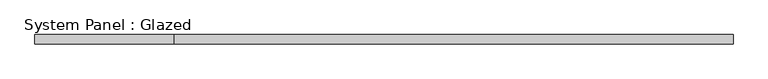
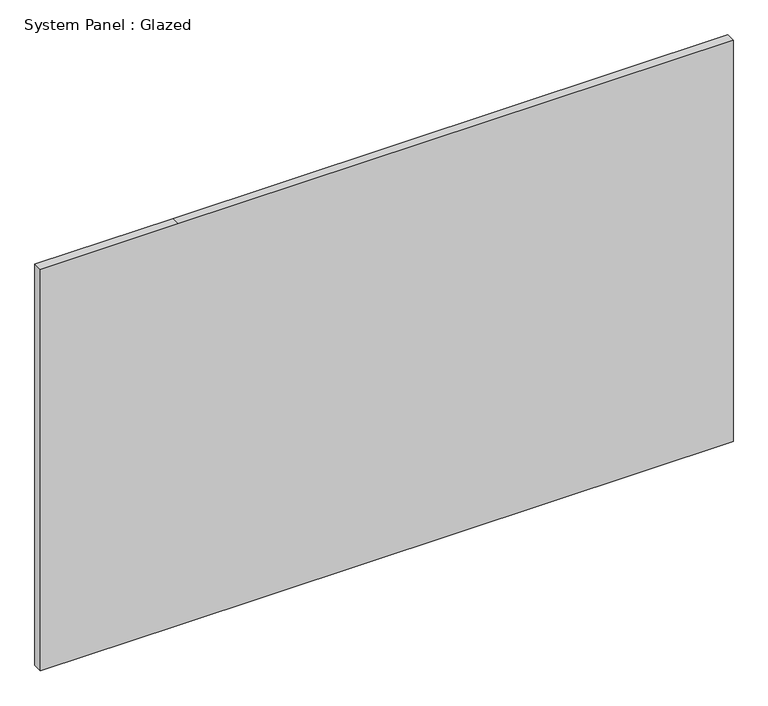
"""IFC4 building model written with IfcOpenShell, lengths in millimetres: plate geometry, System Panel : Glazed."""

from ifc_helpers import new_model, si_unit, frame, origin, place, context, project, spatial, polyline, outline, extrude, source, transform, mapped, element, save


def system_panel_glazed_1ad7f91b(model_context):
    return source(origin(), model_context, "Body", "SweptSolid", [
        extrude(outline(polyline([(0.0, -932.5428571), (0.0, -560.6142857), (0.0, 932.5428571), (1143.0, 932.5428571), (1143.0, -560.6142857), (1143.0, -932.5428571), (0.0, -932.5428571)])), frame((0.0, -12.7, 0.0), z_axis=(0.0, 1.0, 0.0), x_axis=(0.0, 0.0, 1.0)), (0.0, 0.0, 1.0), 25.4),
    ])


if __name__ == "__main__":
    model = new_model("IFC4")
    model_context = context("Model", 3, world=origin())
    ifc_project = project(units=[si_unit("LENGTHUNIT", "METRE", prefix="MILLI")], contexts=[model_context])
    site = spatial("IfcSite", under=ifc_project)
    building = spatial("IfcBuilding", under=site)
    placement = place(None, origin())
    system_panel_glazed_shape = system_panel_glazed_1ad7f91b(model_context)
    element("IfcPlate", 1, ObjectType="System Panel : Glazed", at=placement, inside=building, context=model_context, shape_type="MappedRepresentation", body=[
        mapped(system_panel_glazed_shape, transform((0.0, 0.0, 0.0), x_axis=(1.0, 0.0, 0.0), y_axis=(0.0, 1.0, 0.0), z_axis=(0.0, 0.0, 1.0))),
    ])
    save(model, "model.ifc")

# Revit data of these elements
# Element 1 (IfcPlate, "System Panel : Glazed")
#   Materials on its faces: "Glass"
# Materials
#   "Glass": class "Glass", colour RGB 218 227 224, transparency 0.85, Description = "Soda Lime Glass", Cost = 0
